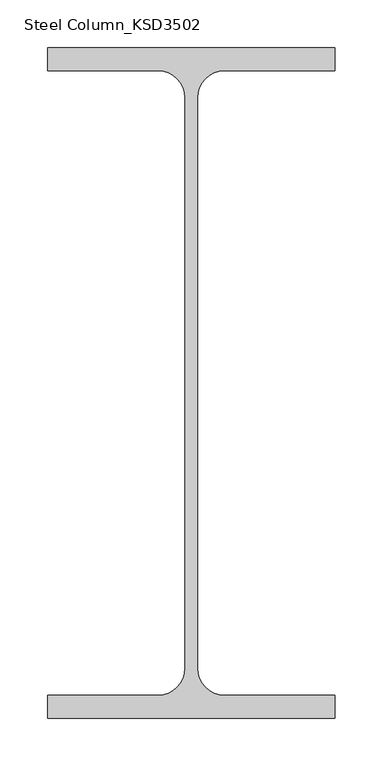
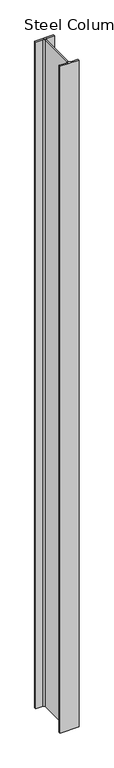
"""IFC4 building model written with IfcOpenShell, lengths in millimetres: column geometry, Steel Column_KSD3502 : H_SC_ASC_H-700×300x13x24."""

from ifc_helpers import new_model, si_unit, point, frame, frame_2d, origin, place, context, project, spatial, polyline, circle_curve, trimmed, segment, composite_curve, outline, extrude, source, transform, mapped, element, save


def steel_column_ksd3502_8461dad7(model_context):
    return source(origin(), model_context, "Body", "SweptSolid", [
        extrude(outline(composite_curve([segment(polyline([(150.0, 350.0), (150.0, 326.0), (34.5, 326.0)]), True, "CONTINUOUS"), segment(trimmed(circle_curve(frame_2d((34.5, 298.0)), 28.0), [point((34.5, 326.0))], [point((6.5, 298.0))], True, "CARTESIAN"), True, "CONTINUOUS"), segment(polyline([(6.5, 298.0), (6.5, -298.0)]), True, "CONTINUOUS"), segment(trimmed(circle_curve(frame_2d((34.5, -298.0)), 28.0), [point((6.5, -298.0))], [point((34.5, -326.0))], True, "CARTESIAN"), True, "CONTINUOUS"), segment(polyline([(34.5, -326.0), (150.0, -326.0), (150.0, -350.0), (-150.0, -350.0), (-150.0, -326.0), (-34.5, -326.0)]), True, "CONTINUOUS"), segment(trimmed(circle_curve(frame_2d((-34.5, -298.0)), 28.0), [point((-34.5, -326.0))], [point((-6.5, -298.0))], True, "CARTESIAN"), True, "CONTINUOUS"), segment(polyline([(-6.5, -298.0), (-6.5, 298.0)]), True, "CONTINUOUS"), segment(trimmed(circle_curve(frame_2d((-34.5, 298.0)), 28.0), [point((-6.5, 298.0))], [point((-34.5, 326.0))], True, "CARTESIAN"), True, "CONTINUOUS"), segment(polyline([(-34.5, 326.0), (-150.0, 326.0), (-150.0, 350.0), (150.0, 350.0)]), True, "CONTINUOUS")], self_intersect=False)), frame((0.0, 0.0, 685.9720055), z_axis=(0.0, 0.0, 1.0), x_axis=(1.0, 0.0, 0.0)), (0.0, 0.0, 1.0), 11224.0),
    ])


if __name__ == "__main__":
    model = new_model("IFC4")
    model_context = context("Model", 3, world=origin())
    ifc_project = project(units=[si_unit("LENGTHUNIT", "METRE", prefix="MILLI")], contexts=[model_context])
    site = spatial("IfcSite", under=ifc_project)
    building = spatial("IfcBuilding", under=site)
    placement = place(None, origin())
    steel_column_ksd3502_shape = steel_column_ksd3502_8461dad7(model_context)
    element("IfcColumn", 1, ObjectType="Steel Column_KSD3502 : H_SC_ASC_H-700×300x13x24", at=placement, inside=building, context=model_context, shape_type="MappedRepresentation", body=[
        mapped(steel_column_ksd3502_shape, transform((0.0, 0.0, 0.0), x_axis=(1.0, 0.0, 0.0), y_axis=(0.0, 1.0, 0.0), z_axis=(0.0, 0.0, 1.0))),
    ])
    save(model, "model.ifc")

# Revit data of these elements
# Type "Steel Column_KSD3502 : H_SC_ASC_H-700×300x13x24"
#   Width = 30.0 cm
#   Web Thickness = 1.3 cm
#   Web Fillet = 2.8 cm
#   Warping Constant = 12338400.0 cm⁶
#   Torsional Moment of Inertia = 325.986 cm⁴
#   Section Area = 235.5 cm²
#   Plastic Modulus weak axis = 1120.0 cm³
#   Plastic Modulus strong axis = 6460.0 cm³
#   Perimeter = 1.27 m²/m
#   Nominal Weight = 185.00 kgf/m
#   Moment of Inertia weak axis = 10800.00 cm⁴
#   Moment of Inertia strong axis = 201000.00 cm⁴
#   Height = 70.0 cm
#   Flange Thickness = 2.4 cm
#   Elastic Modulus weak axis = 722.0 cm³
#   Elastic Modulus strong axis = 5760.0 cm³
#   Centroid Vertical = 35.0 cm
#   Centroid Horizontal = 15.0 cm
#   Bolt Spacing = 13.97 cm
#   Structural Material [instance default] = Steel, 45-345
#   Section Name Key = ""
#   Assembly Code = ""
# Element 1 (IfcColumn, "Steel Column_KSD3502 : H_SC_ASC_H-700×300x13x24")
#   Structural Material = A03AD029-00008_Anchor Bolt (Installation only)_M36
#   Materials on its faces: "A03AD029-00008_Anchor Bolt (Installation only)_M36"
# Materials
#   "Steel, 45-345": class "Metal", colour RGB 189 187 185, transparency 0, Description = "Steel 345 MPa", Cost = 0
#   "A03AD029-00008_Anchor Bolt (Installation only)_M36": class "Unassigned", colour RGB 84 83 81, transparency 0, Cost = 0
